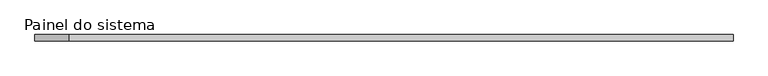
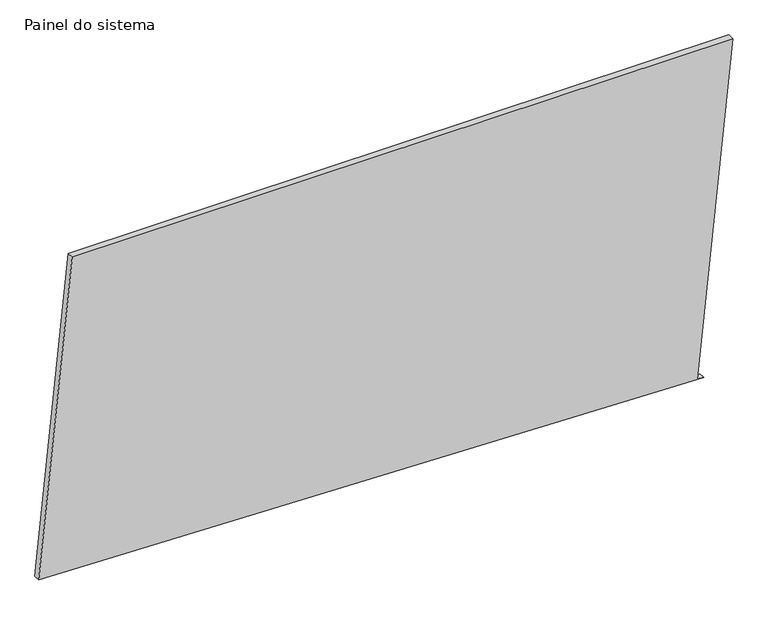
"""IFC4 building model written with IfcOpenShell, lengths in millimetres: plate geometry, Painel do sistema : Envidraçado."""

import ifcopenshell
import ifcopenshell.guid

model = None  # the IFC model being written
_history = None  # IfcOwnerHistory: only IFC2X3 demands one
_inside = {}  # id of a spatial element -> (the spatial element, [elements in it])
_under = {}  # id of a project, library or spatial element -> (it, [spatial elements below it])
_declared = {}  # id of a project -> (the project, [libraries it declares])
_typed = {}  # id of a type object -> (the type object, [elements of that type])
_made_of = {}  # id of a material, layer set ... -> (it, [elements and type objects made of it])


def new_model(schema):
    """Start an empty IFC model of exactly this schema.

    Asked for "IFC4X3", IfcOpenShell would pick the latest addendum, in which some entities
    have other attributes; the version numbers below select the first issue.
    IFC2X3 requires an IfcOwnerHistory on every rooted entity: one is made here for all.
    """
    global model, _history
    if schema == "IFC4X3":
        model = ifcopenshell.file(schema_version=(4, 3, 0, 0))
    else:
        model = ifcopenshell.file(schema=schema)
    _inside.clear()
    _under.clear()
    _declared.clear()
    _typed.clear()
    _made_of.clear()
    _history = None
    if model.schema == "IFC2X3":
        org = make("IfcOrganization", Name="unknown")
        user = make(
            "IfcPersonAndOrganization",
            ThePerson=make("IfcPerson", FamilyName="unknown"),
            TheOrganization=org,
        )
        app = make(
            "IfcApplication",
            ApplicationDeveloper=org,
            Version="unknown",
            ApplicationFullName="unknown",
            ApplicationIdentifier="unknown",
        )
        _history = make(
            "IfcOwnerHistory",
            OwningUser=user,
            OwningApplication=app,
            ChangeAction="ADDED",
            CreationDate=0,
        )
    return model


def make(cls, **values):
    """One entity of the class cls with the attributes given. An attribute that is None is left unset."""
    return model.create_entity(
        cls, **{name: value for name, value in values.items() if value is not None}
    )


def rooted(cls, **values):
    """An entity with a GlobalId (a new one), such as an element, a storey or a relation."""
    return make(cls, GlobalId=ifcopenshell.guid.new(), OwnerHistory=_history, **values)


def si_unit(unit_type, name, prefix=None):
    """IfcSIUnit, for example si_unit("LENGTHUNIT", "METRE", prefix="MILLI")."""
    return make("IfcSIUnit", UnitType=unit_type, Prefix=prefix, Name=name)


def assignment(units):
    """IfcUnitAssignment: the units of a project."""
    return None if units is None else make("IfcUnitAssignment", Units=units)


def point(xyz):
    """IfcCartesianPoint."""
    return None if xyz is None else make("IfcCartesianPoint", Coordinates=xyz)


def direction(xyz):
    """IfcDirection."""
    return None if xyz is None else make("IfcDirection", DirectionRatios=xyz)


def frame(location, z_axis=None, x_axis=None):
    """IfcAxis2Placement3D, a coordinate frame: its origin and axes. An axis left out is left unset."""
    return make(
        "IfcAxis2Placement3D",
        Location=point(location),
        Axis=direction(z_axis),
        RefDirection=direction(x_axis),
    )


def origin():
    """The frame at (0, 0, 0) with its axes left unset."""
    return frame((0.0, 0.0, 0.0))


def place(relative_to, where):
    """IfcLocalPlacement: puts the frame where relative to a parent placement (None: the world)."""
    return make(
        "IfcLocalPlacement", PlacementRelTo=relative_to, RelativePlacement=where
    )


def context(
    kind, dimensions, precision=None, world=None, true_north=None, identifier=None
):
    """IfcGeometricRepresentationContext, for example the 3D "Model" context."""
    return make(
        "IfcGeometricRepresentationContext",
        ContextIdentifier=identifier,
        ContextType=kind,
        CoordinateSpaceDimension=dimensions,
        Precision=precision,
        WorldCoordinateSystem=world,
        TrueNorth=true_north,
    )


def project(units=None, contexts=None):
    """IfcProject with its units and contexts."""
    return rooted(
        "IfcProject",
        Name="project",
        RepresentationContexts=contexts,
        UnitsInContext=assignment(units),
    )


def spatial(cls, under=None, at=None, **own):
    """A site, building, storey or space (cls), placed at a placement, below another one or the project."""
    s = rooted(cls, ObjectPlacement=at, **own)
    if under is not None:
        _under.setdefault(under.id(), (under, []))[1].append(s)
    return s


def polyline(points):
    """IfcPolyline through the points."""
    return make("IfcPolyline", Points=[point(p) for p in points])


def outline(outer, holes=None, kind="AREA"):
    """IfcArbitraryClosedProfileDef: a profile drawn as a closed curve; with holes, ...WithVoids."""
    if holes is None:
        return make("IfcArbitraryClosedProfileDef", ProfileType=kind, OuterCurve=outer)
    return make(
        "IfcArbitraryProfileDefWithVoids",
        ProfileType=kind,
        OuterCurve=outer,
        InnerCurves=holes,
    )


def extrude(swept, where, along, depth):
    """IfcExtrudedAreaSolid: the profile swept, set in the frame where, extruded along a direction by depth."""
    return make(
        "IfcExtrudedAreaSolid",
        SweptArea=swept,
        Position=where,
        ExtrudedDirection=direction(along),
        Depth=depth,
    )


def shape(context_of_items, identifier, shape_type, items):
    """IfcShapeRepresentation: the items that make up one representation, for example the "Body"."""
    return make(
        "IfcShapeRepresentation",
        ContextOfItems=context_of_items,
        RepresentationIdentifier=identifier,
        RepresentationType=shape_type,
        Items=items,
    )


def source(mapping_origin, context_of_items, identifier, shape_type, items):
    """IfcRepresentationMap: a shape defined once, which mapped items show again and again."""
    return make(
        "IfcRepresentationMap",
        MappingOrigin=mapping_origin,
        MappedRepresentation=shape(context_of_items, identifier, shape_type, items),
    )


def transform(
    local_origin,
    x_axis=None,
    y_axis=None,
    z_axis=None,
    scale=None,
    scale2=None,
    scale3=None,
    uniform=True,
):
    """IfcCartesianTransformationOperator3D, or its non-uniform kind. x_axis, y_axis, z_axis: its Axis1, 2, 3."""
    if uniform:
        return make(
            "IfcCartesianTransformationOperator3D",
            Axis1=direction(x_axis),
            Axis2=direction(y_axis),
            LocalOrigin=point(local_origin),
            Scale=scale,
            Axis3=direction(z_axis),
        )
    return make(
        "IfcCartesianTransformationOperator3DnonUniform",
        Axis1=direction(x_axis),
        Axis2=direction(y_axis),
        LocalOrigin=point(local_origin),
        Scale=scale,
        Axis3=direction(z_axis),
        Scale2=scale2,
        Scale3=scale3,
    )


def mapped(mapping_source, mapping_target):
    """IfcMappedItem: shows the shape of a source again, moved by a transform."""
    return make(
        "IfcMappedItem", MappingSource=mapping_source, MappingTarget=mapping_target
    )


def made_of(thing, what):
    """Note that an element or type object is made of a material, layer set ...; save() writes the relation."""
    if what is not None:
        _made_of.setdefault(what.id(), (what, []))[1].append(thing)
    return thing


def element(
    cls,
    number,
    at=None,
    inside=None,
    cuts=None,
    type_object=None,
    material=None,
    context=None,
    identifier="Body",
    shape_type=None,
    held_by="IfcProductDefinitionShape",
    body=None,
    shapes=None,
    **own,
):
    """One element of the class cls, such as IfcWall. Its Tag is "e" and its number.

    at: its placement. inside: the storey or other place that contains it. cuts: it is an
    opening in that element (IfcRelVoidsElement). A single representation is given by context,
    identifier, shape_type and body (its items); several are given by shapes. held_by: the class
    of the entity that holds the representations. save() writes the other relations.
    """
    e = rooted(cls, Tag="e%d" % number, ObjectPlacement=at, **own)
    if body is not None:
        shapes = [shape(context, identifier, shape_type, body)]
    if shapes is not None:
        e.Representation = make(held_by, Representations=shapes)
    if inside is not None:
        _inside.setdefault(inside.id(), (inside, []))[1].append(e)
    if cuts is not None:
        rooted(
            "IfcRelVoidsElement", RelatingBuildingElement=cuts, RelatedOpeningElement=e
        )
    if type_object is not None:
        _typed.setdefault(type_object.id(), (type_object, []))[1].append(e)
    return made_of(e, material)


def aggregate(whole, parts):
    """IfcRelAggregates: a whole, such as a stair, and the parts it consists of."""
    return rooted("IfcRelAggregates", RelatingObject=whole, RelatedObjects=parts)


def save(model, path):
    """Write the relations noted so far, then the file.

    IfcRelAggregates (storeys below a building ...), IfcRelContainedInSpatialStructure (elements
    in a storey), IfcRelDefinesByType, IfcRelAssociatesMaterial and IfcRelDeclares: one each for
    every whole, place, type object, material and project.
    """
    for whole, parts in _under.values():
        aggregate(whole, parts)
    for where, things in _inside.values():
        rooted(
            "IfcRelContainedInSpatialStructure",
            RelatedElements=things,
            RelatingStructure=where,
        )
    for kind, things in _typed.values():
        rooted("IfcRelDefinesByType", RelatedObjects=things, RelatingType=kind)
    for what, things in _made_of.values():
        rooted("IfcRelAssociatesMaterial", RelatedObjects=things, RelatingMaterial=what)
    for by, libraries in _declared.values():
        rooted("IfcRelDeclares", RelatingContext=by, RelatedDefinitions=libraries)
    model.write(path)


def painel_do_sistema_23c5740b(model_context):
    return source(origin(), model_context, "Body", "SweptSolid", [
        extrude(outline(polyline([(0.0, 1233.0579279), (2.5300763, 1208.1862831), (1350.6532848, 1345.3245626), (1350.6532848, -1215.4519521), (73.9544594, -1345.3245626), (0.0, 1233.0579279)])), frame((0.0, 24.5, 0.0), z_axis=(0.0, 1.0, 0.0), x_axis=(0.0, 0.0, 1.0)), (0.0, 0.0, 1.0), 25.0),
    ])


if __name__ == "__main__":
    model = new_model("IFC4")
    model_context = context("Model", 3, world=origin())
    ifc_project = project(units=[si_unit("LENGTHUNIT", "METRE", prefix="MILLI")], contexts=[model_context])
    site = spatial("IfcSite", under=ifc_project)
    building = spatial("IfcBuilding", under=site)
    placement = place(None, origin())
    painel_do_sistema_shape = painel_do_sistema_23c5740b(model_context)
    element("IfcPlate", 1, ObjectType="Painel do sistema : Envidraçado", at=placement, inside=building, context=model_context, shape_type="MappedRepresentation", body=[
        mapped(painel_do_sistema_shape, transform((0.0, 0.0, 0.0), x_axis=(1.0, 0.0, 0.0), y_axis=(0.0, 1.0, 0.0), z_axis=(0.0, 0.0, 1.0))),
    ])
    save(model, "model.ifc")

# Revit data of these elements
# Type "Painel do sistema : Envidraçado"
#   Construction Type Id = "GSP4R"
#   Analytic Construction = "Vidraça única Pilkington 1/8 pol"
#   Visual Light Transmittance = 0.9
#   Solar Heat Gain Coefficient = 0.86
#   Heat Transfer Coefficient (U) = 6.7069 W/(m²·K)
# Element 1 (IfcPlate, "Painel do sistema : Envidraçado")
#   Materials on its faces: "Vidro"
# Materials
#   "Vidro": class "Vidro", colour RGB 0 128 192, transparency 0.9, Description = "Vidro de sílica", Cost = 0
